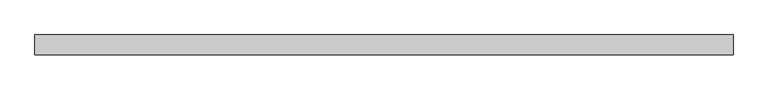
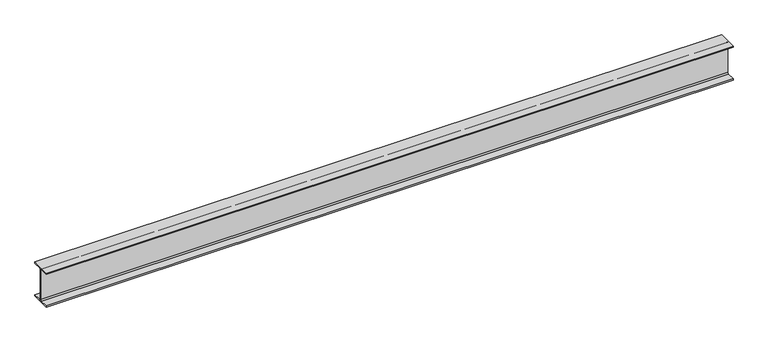
"""IFC4 building model written with IfcOpenShell, lengths in millimetres: beam geometry, Old_Steel Beam_H-KSD3502 : H_SB_ASB_H-350×175x7x11."""

from ifc_helpers import new_model, si_unit, point, frame, frame_2d, origin, place, context, project, spatial, polyline, circle_curve, trimmed, segment, composite_curve, outline, extrude, source, transform, mapped, element, save


def beam_550b7d4d(model_context):
    return source(origin(), model_context, "Body", "SweptSolid", [
        extrude(outline(composite_curve([segment(polyline([(82.5, -141.5), (82.5, -151.7), (-82.5, -151.7), (-82.5, -141.5), (-11.9, -141.5)]), True, "CONTINUOUS"), segment(trimmed(circle_curve(frame_2d((-11.9, -132.6)), 8.9), [point((-11.9, -141.5))], [point((-3.0, -132.6))], True, "CARTESIAN"), True, "CONTINUOUS"), segment(polyline([(-3.0, -132.6), (-3.0, 132.6)]), True, "CONTINUOUS"), segment(trimmed(circle_curve(frame_2d((-11.9, 132.6)), 8.9), [point((-3.0, 132.6))], [point((-11.9, 141.5))], True, "CARTESIAN"), True, "CONTINUOUS"), segment(polyline([(-11.9, 141.5), (-82.5, 141.5), (-82.5, 151.7), (82.5, 151.7), (82.5, 141.5), (11.9, 141.5)]), True, "CONTINUOUS"), segment(trimmed(circle_curve(frame_2d((11.9, 132.6)), 8.9), [point((11.9, 141.5))], [point((3.0, 132.6))], True, "CARTESIAN"), True, "CONTINUOUS"), segment(polyline([(3.0, 132.6), (3.0, -132.6)]), True, "CONTINUOUS"), segment(trimmed(circle_curve(frame_2d((11.9, -132.6)), 8.9), [point((3.0, -132.6))], [point((11.9, -141.5))], True, "CARTESIAN"), True, "CONTINUOUS"), segment(polyline([(11.9, -141.5), (82.5, -141.5)]), True, "CONTINUOUS")], self_intersect=False)), frame((-2920.1382551, 0.0, 0.0), z_axis=(1.0, 0.0, 0.0), x_axis=(0.0, 1.0, 0.0)), (0.0, 0.0, 1.0), 5810.1551285),
    ])


if __name__ == "__main__":
    model = new_model("IFC4")
    model_context = context("Model", 3, world=origin())
    ifc_project = project(units=[si_unit("LENGTHUNIT", "METRE", prefix="MILLI")], contexts=[model_context])
    site = spatial("IfcSite", under=ifc_project)
    building = spatial("IfcBuilding", under=site)
    placement = place(None, origin())
    beam_shape = beam_550b7d4d(model_context)
    element("IfcBeam", 1, ObjectType="Old_Steel Beam_H-KSD3502 : H_SB_ASB_H-350×175x7x11", at=placement, inside=building, context=model_context, shape_type="MappedRepresentation", body=[
        mapped(beam_shape, transform((0.0, 0.0, 0.0), x_axis=(1.0, 0.0, 0.0), y_axis=(0.0, 1.0, 0.0), z_axis=(0.0, 0.0, 1.0))),
    ])
    save(model, "model.ifc")

# Revit data of these elements
# Type "Old_Steel Beam_H-KSD3502 : H_SB_ASB_H-350×175x7x11"
#   Width = 17.5 cm
#   Web Thickness = 0.7 cm
#   Web Fillet = 1.4 cm
#   Warping Constant = 282290.0 cm⁶
#   Torsional Moment of Inertia = 19.4042 cm⁴
#   Torsional Modulus = 1.0 cm³
#   Section Area = 63.14 cm²
#   Plastic Modulus weak axis = 174.0 cm³
#   Plastic Modulus strong axis = 868.0 cm³
#   Perimeter = 1.36 m²/m
#   Nominal Weight = 49.60 kgf/m
#   Moment of Inertia weak axis = 984.00 cm⁴
#   Moment of Inertia strong axis = 13600.00 cm⁴
#   Height = 35.0 cm
#   Flange Thickness = 1.1 cm
#   Elastic Modulus weak axis = 112.0 cm³
#   Elastic Modulus strong axis = 775.0 cm³
#   Centroid Vertical = 17.5 cm
#   Centroid Horizontal = 8.75 cm
#   Length [instance default] = 1.5240 m
#   Structural Material [instance default] = Steel, 45-345
#   Assembly Code = ""
# Element 1 (IfcBeam, "Old_Steel Beam_H-KSD3502 : H_SB_ASB_H-350×175x7x11")
#   Structural Material = none
# Materials
#   "Steel, 45-345": class "Metal", colour RGB 189 187 185, transparency 0, Description = "Steel 345 MPa", Cost = 0
